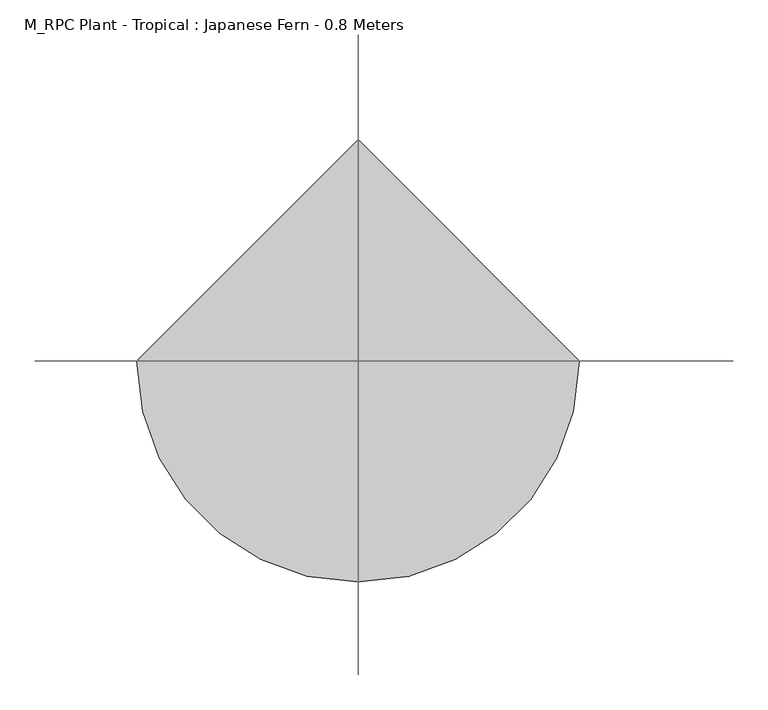
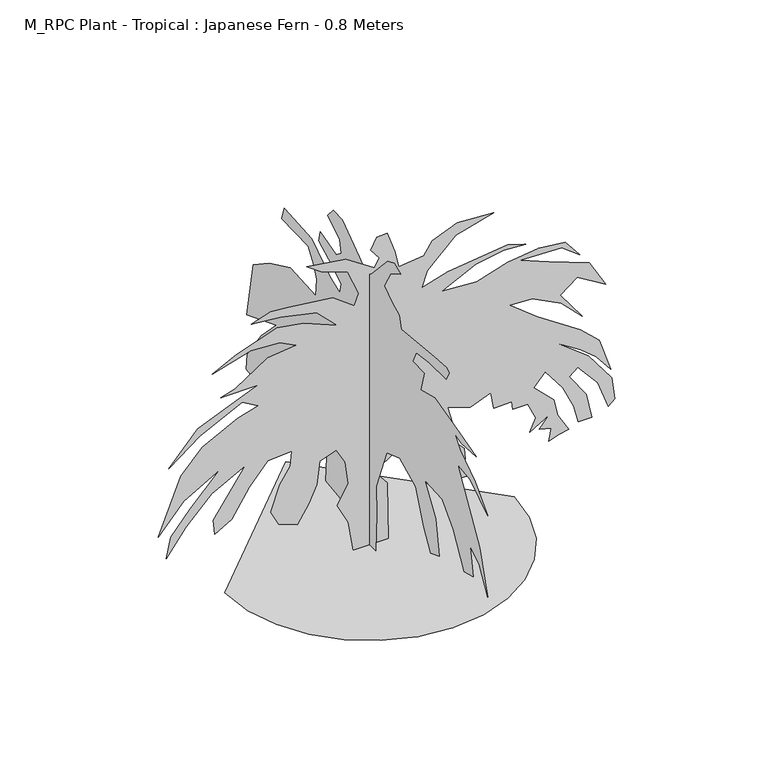
"""IFC4 building model written with IfcOpenShell, lengths in millimetres: geographic element geometry, M_RPC Plant - Tropical : Japanese Fern - 0.8 Meters."""

from ifc_helpers import new_model, si_unit, origin, place, context, project, spatial, triangles, source, transform, mapped, element, save


def m_rpc_plant_tropical_japanese_fern_0_8_meters_89f61e38(model_context):
    return source(origin(), model_context, "Body", "Tessellation", [
        triangles([(-356.9816259, 0.0, 2.46e-05), (-347.538961, -81.8417886, 2.46e-05), (-320.6483422, -157.0003733, 2.46e-05), (-278.4590569, -223.3224515, 2.46e-05), (-223.1257884, -278.6557201, 2.46e-05), (-156.8037101, -320.8450235, 2.46e-05), (-81.6451164, -347.7356423, 2.46e-05), (0.1966867, -357.1783072, 2.46e-05), (82.0384609, -347.7356423, 2.46e-05), (157.1970364, -320.8450235, 2.46e-05), (223.5191146, -278.6557201, 2.46e-05), (278.8523832, -223.3224515, 2.46e-05), (321.0417048, -157.0003733, 2.46e-05), (347.9323236, -81.8417886, 2.46e-05), (357.3749886, 3.12e-05, 2.46e-05), (0.1966242, 357.1783072, 2.46e-05), (-39.591288, 2.4e-05, 3.8e-06), (-52.3886082, 2.53e-05, 77.2092589), (-79.4701856, 2.33e-05, 129.9044073), (-51.8286088, 1.92e-05, 179.0246285), (-59.6237998, 1.61e-05, 237.2005651), (-81.0099172, 1.47e-05, 275.3224025), (-121.8640096, 1.74e-05, 260.7322683), (-129.4650627, 2.12e-05, 202.3781994), (-150.0026445, 2.47e-05, 159.3985009), (-177.3082362, 2.85e-05, 114.8257492), (-224.1652416, 2.95e-05, 132.5502668), (-243.9444304, 2.81e-05, 171.1790318), (-221.0799103, 2.33e-05, 234.4691003), (-195.0511394, 1.98e-05, 273.6130591), (-191.2119478, 1.74e-05, 311.3276902), (-250.2614867, 2.02e-05, 307.4210246), (-296.6350369, 2.54e-05, 254.2280142), (-339.5123071, 3.14e-05, 185.9592888), (-381.4722822, 3.47e-05, 161.1515734), (-385.2696158, 3.25e-05, 199.7619347), (-305.7070304, 2.23e-05, 313.25835), (-389.2322737, 2.86e-05, 269.5890678), (-451.6135314, 3.51e-05, 205.2877965), (-501.5068159, 4.12e-05, 139.8979924), (-490.5788492, 3.76e-05, 191.9816683), (-441.6242065, 3.21e-05, 249.0544201), (-368.8616057, 2.43e-05, 325.6103577), (-458.3148665, 3.13e-05, 274.3943886), (-521.6481374, 3.83e-05, 202.3696607), (-465.4295122, 2.75e-05, 342.7516442), (-412.306919, 2.18e-05, 399.0182679), (-325.1523188, 1.53e-05, 444.1942168), (-273.6057376, 1.22e-05, 459.1648873), (-314.0723265, 1.26e-05, 482.4155394), (-418.6162359, 2.03e-05, 430.012924), (-495.2054927, 2.71e-05, 372.3782879), (-423.1042251, 1.92e-05, 451.5675676), (-315.4003341, 1.18e-05, 496.7035117), (-275.4804052, 9.1e-06, 512.7808371), (-366.2136206, 1.31e-05, 512.5835017), (-331.2056557, 1.09e-05, 523.2341598), (-250.2614867, 4.2e-06, 575.8901027), (-180.8079499, 7e-07, 584.7194329), (-221.0799103, 1.2e-06, 605.0713883), (-292.4937199, 4.1e-06, 609.4207232), (-387.4135983, 9.9e-06, 581.7274281), (-328.4856545, 5.5e-06, 612.0154049), (-227.295374, -1e-06, 646.7967121), (-161.5869029, -3.2e-06, 635.7193359), (-78.621382, -4.8e-06, 600.674055), (-129.4533356, -5.6e-06, 651.5887161), (-219.3260566, -2.8e-06, 670.7326784), (-291.1150432, -1e-07, 678.0232944), (-243.6241556, -3.1e-06, 694.5326792), (-199.2876722, -4.8e-06, 690.5139565), (-89.7989701, -8.8e-06, 676.7513517), (-37.2379591, -8.7e-06, 637.1700468), (-25.5654385, -1.1e-05, 666.3513325), (-53.2067405, -1.36e-05, 730.9165775), (-118.8594782, -1.21e-05, 754.0578976), (-153.9631858, -1.22e-05, 780.1592113), (-58.1566019, -1.55e-05, 766.6525503), (12.3701786, -1.58e-05, 718.8793036), (24.5030987, -1.76e-05, 741.3032982), (3.6158409, -1.84e-05, 768.4872494), (18.7047597, -2.07e-05, 796.1618683), (43.7640938, -2.19e-05, 798.4898512), (62.816342, -1.95e-05, 744.3539114), (72.129132, -1.74e-05, 701.4126371), (134.0245409, -2.04e-05, 707.8552671), (155.3583768, -2.33e-05, 739.3059637), (216.6393747, -2.75e-05, 765.5672241), (307.1003683, -3.11e-05, 759.7325512), (213.1465828, -2.54e-05, 733.5272467), (143.1669335, -1.83e-05, 665.9780268), (130.1258781, -1.53e-05, 625.1620588), (193.29407, -1.93e-05, 645.9246723), (342.1190157, -2.69e-05, 663.433996), (386.0096143, -2.8e-05, 650.2686659), (331.6310294, -2.58e-05, 653.215361), (262.3572055, -2.2e-05, 640.2313425), (179.4618111, -1.6e-05, 599.1567421), (265.035058, -1.94e-05, 594.3860667), (342.0896934, -2.42e-05, 617.5967503), (417.9909471, -2.81e-05, 628.4153486), (483.3268573, -3.05e-05, 620.5620489), (520.1241752, -2.95e-05, 575.8901027), (475.7348788, -2.95e-05, 609.4687217), (372.9456588, -2.52e-05, 612.3860945), (441.3349073, -2.65e-05, 584.6447645), (542.8041498, -2.87e-05, 546.4048021), (584.2227699, -2.63e-05, 476.0742113), (513.9028253, -2.58e-05, 519.0714778), (472.0308898, -2.2e-05, 486.8048427), (525.9615005, -2e-05, 412.4742416), (473.4335295, -2.08e-05, 465.0022127), (402.3962957, -1.99e-05, 501.5674953), (346.6470097, -1.76e-05, 504.9195073), (415.0709218, -1.74e-05, 450.4102255), (520.5801793, -1.78e-05, 379.9196154), (568.2414416, -1.72e-05, 335.1356847), (596.0814211, -1.33e-05, 249.2213612), (560.7561427, -1.45e-05, 294.909034), (522.6121774, -1.47e-05, 326.2076686), (462.342891, -1.43e-05, 363.9543108), (540.550799, -1.42e-05, 304.5037063), (599.2467439, -1.21e-05, 226.7565805), (605.6067481, -9e-06, 169.6256927), (590.1587448, -7.5e-06, 155.6795782), (563.8974481, -1.05e-05, 225.714711), (514.2895022, -1.18e-05, 284.0770462), (493.1588516, -9.9e-06, 266.7677284), (536.2361641, -8.1e-06, 205.2771322), (549.3054608, -4.8e-06, 141.0889262), (516.425491, -3.3e-06, 140.2646579), (505.3241701, -5.5e-06, 185.108614), (477.6415575, -7.8e-06, 243.2032329), (434.3535748, -9.2e-06, 299.3437015), (405.9722766, -6.1e-06, 268.3197412), (455.9268946, -5.4e-06, 219.8784575), (465.4788915, -3.2e-06, 174.9152863), (492.2202098, -1.7e-06, 130.1460077), (468.8415496, -3e-07, 124.1884135), (442.7215596, 1.3e-06, 116.1070845), (449.5455617, -8e-07, 146.8782531), (419.662938, 0.0, 155.0435705), (444.2522438, -2.8e-06, 184.860882), (396.2229444, 1e-06, 156.0027779), (410.9322573, -1.6e-06, 188.0872839), (391.7616251, -3.2e-06, 229.804832), (353.6443296, -1.6e-06, 230.0109786), (351.7750033, -2.7e-06, 250.1848198), (307.1003683, -7e-07, 249.0597613), (300.2817075, -2.9e-06, 291.6023862), (248.7385418, 5e-07, 272.405066), (193.29407, 1.9e-06, 289.9143715), (210.8028487, 4.9e-06, 225.714711), (209.5596469, 6.7e-06, 196.5163297), (234.147899, 7.2e-06, 170.2702392), (237.0660348, 8.8e-06, 141.0889262), (219.1519212, 1.04e-05, 127.6382756), (249.9017521, 1.1e-05, 94.9585752), (191.3132679, 1.34e-05, 97.4711035), (201.263133, 1.05e-05, 139.9955973), (173.9058276, 1.05e-05, 159.8089046), (182.4415529, 8.6e-06, 185.1459482), (114.684288, 1.2e-05, 178.0643492), (99.9141775, 1.12e-05, 202.3696607), (152.4405135, 7.1e-06, 231.5509645), (87.6747175, 9.8e-06, 234.8944377), (12.4554318, 1.6e-05, 186.0566121), (44.4696966, 1.69e-05, 146.9251888), (47.3878233, 1.91e-05, 0.0), (0.1988968, 28.0250381, 3.7e-06), (0.1989024, 23.3153101, 131.4809371), (0.1989043, 63.1703357, 135.2526637), (0.1989031, 125.3580096, 45.104755), (0.1989061, 186.8720783, 53.6724779), (0.1989088, 182.1083611, 118.7774792), (0.1989112, 144.4259864, 212.5160617), (0.1989072, 143.3849253, 265.1541278), (0.1989091, 175.7563505, 275.9837175), (0.1989147, 237.6858916, 199.7619347), (0.198915, 302.7357001, 140.1214617), (0.1989165, 331.3730146, 147.3601187), (0.1989186, 325.3463476, 199.5424713), (0.1989213, 363.9222997, 223.1101825), (0.1989223, 429.8262348, 180.7067569), (0.1989222, 475.8741872, 131.4809371), (0.1989247, 526.6901261, 139.4206596), (0.1989263, 521.9248283, 180.7067569), (0.1989212, 463.1728912, 264.866936), (0.1989213, 397.7889462, 332.7090159), (0.1989246, 523.5141572, 283.9223863), (0.1989299, 495.7835097, 430.9862294), (0.1989289, 428.236906, 476.0608764), (0.1989268, 339.3143177, 517.3488358), (0.1989217, 228.4952462, 512.2821756), (0.1989235, 224.9824519, 557.0447777), (0.1989254, 238.2328241, 586.9834299), (0.198928, 261.7722666, 621.3780602), (0.198933, 375.8342906, 623.7380178), (0.198934, 364.7196347, 657.0846743), (0.1989285, 247.1213622, 649.612674), (0.1989229, 169.3534347, 598.4660866), (0.1989203, 125.6708085, 581.7007582), (0.1989213, 121.2033486, 608.4554114), (0.1989249, 174.1686204, 639.6180079), (0.1989278, 217.0427113, 661.8500084), (0.1989224, 209.1029888, 690.4313307), (0.1989186, 140.9505263, 671.9353666), (0.1989184, 120.1790834, 688.8446543), (0.1989201, 126.4332074, 719.3166315), (0.1989238, 178.9323558, 752.3619255), (0.1989239, 155.1134427, 779.3565714), (0.1989222, 117.0030872, 777.7672062), (0.1989167, 43.7690217, 725.5806387), (0.1989142, 11.282335, 699.1806513), (0.1989139, -10.6222293, 714.4366241), (0.1989141, -78.3121894, 787.2951857), (0.1989134, -106.8948288, 799.9992067), (0.1989117, -133.8897381, 787.2951857), (0.1989124, -91.4905729, 762.6498877), (0.1989115, -63.82447, 714.9192982), (0.198909, -97.1412363, 690.3886734), (0.1989071, -127.8788042, 676.3806622), (0.1989116, -136.2243976, 645.8900087), (0.1988998, -278.3917282, 660.2606432), (0.1988976, -330.7943436, 663.4366848), (0.1988968, -341.9089994, 655.4979979), (0.1989026, -329.2050147, 631.6793936), (0.1989057, -255.7989394, 630.9247158), (0.1989078, -201.4115251, 623.4394169), (0.1989071, -185.4035451, 591.3727332), (0.1989049, -234.4786928, 590.4820899), (0.1989033, -219.4389858, 537.8608106), (0.1989013, -279.9783864, 553.8714612), (0.1988956, -384.8262926, 526.9594774), (0.1988915, -456.2395572, 506.2314912), (0.1988942, -394.0155936, 503.9995053), (0.1988957, -365.7943148, 511.6901696), (0.1988935, -388.4636069, 482.6261733), (0.1988888, -452.284893, 439.6635704), (0.198884, -507.0528437, 383.9622828), (0.1988894, -430.8768974, 431.8128868), (0.198892, -378.3489627, 438.6928811), (0.1988872, -418.3222495, 368.7036212), (0.1988809, -472.1195472, 279.1570521), (0.1988809, -505.8634904, 170.2702392), (0.198879, -470.530182, 233.1083004), (0.1988817, -430.9435721, 256.6434736), (0.1988781, -444.5382365, 186.5443548), (0.1988855, -406.6475987, 176.1064927), (0.198885, -359.3756295, 258.5152162), (0.1988892, -311.2476806, 308.3676965), (0.1988927, -237.3971011, 313.25835), (0.1988874, -284.7437206, 241.0480229), (0.1988892, -298.5170441, 151.7734485), (0.1988901, -261.8053315, 136.5182659), (0.1988937, -232.8570984, 188.3064747), (0.1988926, -197.5672648, 272.0370652), (0.198897, -130.1718691, 304.5676922), (0.1988986, -73.5660583, 284.6663815), (0.1989018, -28.8695723, 170.457437), (0.1988986, -31.953834, 99.3204365), (0.1988944, -26.9829074, 2.55e-05)], [[15, 16, 1], [14, 15, 1], [14, 1, 2], [13, 14, 2], [13, 2, 3], [13, 3, 4], [12, 13, 4], [11, 12, 4], [11, 4, 5], [11, 5, 6], [11, 6, 7], [11, 7, 8], [11, 8, 9], [11, 9, 10], [110, 111, 112], [51, 52, 53], [61, 62, 63], [102, 103, 104], [94, 95, 96], [55, 56, 57], [88, 89, 90], [44, 45, 46], [117, 118, 119], [61, 63, 64], [68, 69, 70], [39, 40, 41], [107, 108, 109], [76, 77, 78], [39, 41, 42], [75, 76, 78], [38, 39, 42], [38, 42, 43], [60, 61, 64], [143, 144, 145], [93, 94, 96], [93, 96, 97], [93, 97, 98], [68, 70, 71], [37, 38, 43], [55, 57, 58], [157, 158, 159], [157, 159, 160], [75, 78, 79], [92, 93, 98], [74, 75, 79], [67, 68, 71], [67, 71, 72], [110, 112, 113], [139, 140, 141], [87, 88, 90], [87, 90, 91], [86, 87, 91], [117, 119, 120], [116, 117, 120], [116, 120, 121], [115, 116, 121], [101, 102, 104], [101, 104, 105], [100, 101, 105], [106, 107, 109], [34, 35, 36], [141, 142, 143], [43, 44, 46], [43, 46, 47], [124, 125, 126], [123, 124, 126], [122, 123, 126], [122, 126, 127], [34, 36, 37], [33, 34, 37], [32, 33, 37], [60, 64, 65], [59, 60, 65], [137, 138, 139], [137, 139, 141], [137, 141, 143], [136, 137, 143], [121, 122, 127], [50, 51, 53], [50, 53, 54], [66, 67, 72], [66, 72, 73], [106, 109, 110], [106, 110, 113], [129, 130, 131], [129, 131, 132], [129, 132, 133], [128, 129, 133], [128, 133, 134], [43, 47, 48], [37, 43, 48], [105, 106, 113], [105, 113, 114], [100, 105, 114], [99, 100, 114], [59, 65, 66], [163, 164, 165], [162, 163, 165], [168, 169, 17], [168, 17, 18], [168, 18, 19], [168, 19, 20], [167, 168, 20], [167, 20, 21], [146, 147, 148], [121, 127, 128], [121, 128, 134], [85, 86, 91], [148, 149, 150], [37, 48, 49], [32, 37, 49], [31, 32, 49], [85, 91, 92], [25, 26, 27], [25, 27, 28], [25, 28, 29], [24, 25, 29], [24, 29, 30], [23, 24, 30], [23, 30, 31], [136, 143, 145], [135, 136, 145], [135, 145, 146], [135, 146, 148], [82, 83, 84], [81, 82, 84], [80, 81, 84], [80, 84, 85], [79, 80, 85], [50, 54, 55], [49, 50, 55], [160, 161, 162], [156, 157, 160], [155, 156, 160], [155, 160, 162], [154, 155, 162], [154, 162, 165], [153, 154, 165], [152, 153, 165], [74, 79, 85], [74, 85, 92], [73, 74, 92], [166, 167, 21], [55, 58, 59], [166, 21, 22], [152, 165, 166], [135, 148, 150], [134, 135, 150], [121, 134, 150], [115, 121, 150], [114, 115, 150], [114, 150, 151], [114, 151, 152], [99, 114, 152], [98, 99, 152], [98, 152, 166], [98, 166, 22], [92, 98, 22], [73, 92, 22], [66, 73, 22], [59, 66, 22], [55, 59, 22], [49, 55, 22], [31, 49, 22], [23, 31, 22], [244, 245, 246], [239, 240, 241], [234, 235, 236], [234, 236, 237], [233, 234, 237], [238, 239, 241], [238, 241, 242], [217, 218, 219], [216, 217, 219], [189, 190, 191], [244, 246, 247], [215, 216, 219], [215, 219, 220], [197, 198, 199], [197, 199, 200], [230, 231, 232], [189, 191, 192], [209, 210, 211], [209, 211, 212], [209, 212, 213], [208, 209, 213], [197, 200, 201], [196, 197, 201], [195, 196, 201], [243, 244, 247], [262, 170, 171], [261, 262, 171], [260, 261, 171], [205, 206, 207], [204, 205, 207], [203, 204, 207], [185, 186, 187], [184, 185, 187], [184, 187, 188], [183, 184, 188], [183, 188, 189], [173, 174, 175], [172, 173, 175], [172, 175, 176], [247, 248, 249], [247, 249, 250], [243, 247, 250], [243, 250, 251], [242, 243, 251], [254, 255, 256], [253, 254, 256], [253, 256, 257], [252, 253, 257], [225, 226, 227], [224, 225, 227], [224, 227, 228], [223, 224, 228], [223, 228, 229], [223, 229, 230], [180, 181, 182], [179, 180, 182], [189, 192, 193], [189, 193, 194], [252, 257, 258], [203, 207, 208], [242, 251, 252], [208, 213, 214], [203, 208, 214], [183, 189, 194], [182, 183, 194], [179, 182, 194], [178, 179, 194], [177, 178, 194], [195, 201, 202], [194, 195, 202], [177, 194, 202], [237, 238, 242], [237, 242, 252], [233, 237, 252], [232, 233, 252], [232, 252, 258], [230, 232, 258], [230, 258, 259], [223, 230, 259], [221, 222, 223], [221, 223, 259], [220, 221, 259], [215, 220, 259], [214, 215, 259], [203, 214, 259], [202, 203, 259], [177, 202, 259], [177, 259, 260], [176, 177, 260], [172, 176, 260], [172, 260, 171]], closed=False),
    ])


if __name__ == "__main__":
    model = new_model("IFC4")
    model_context = context("Model", 3, world=origin())
    ifc_project = project(units=[si_unit("LENGTHUNIT", "METRE", prefix="MILLI")], contexts=[model_context])
    site = spatial("IfcSite", under=ifc_project)
    building = spatial("IfcBuilding", under=site)
    placement = place(None, origin())
    m_rpc_plant_tropical_japanese_fern_0_8_meters_shape = m_rpc_plant_tropical_japanese_fern_0_8_meters_89f61e38(model_context)
    element("IfcGeographicElement", 1, ObjectType="M_RPC Plant - Tropical : Japanese Fern - 0.8 Meters", at=placement, inside=building, context=model_context, shape_type="MappedRepresentation", body=[
        mapped(m_rpc_plant_tropical_japanese_fern_0_8_meters_shape, transform((0.0, 0.0, 0.0), x_axis=(1.0, 0.0, 0.0), y_axis=(0.0, 1.0, 0.0), z_axis=(0.0, 0.0, 1.0))),
    ])
    save(model, "model.ifc")

# Revit data of these elements
# Type "M_RPC Plant - Tropical : Japanese Fern - 0.8 Meters"
#   built-in parameter 1005198 = "{2, 15},{39, RPC-16-G1GK-JAPX-7J4P-Q000-ST1L-LVER-AU},{1, 0},{1, 0},{2, 35},{1, 8},{5, Color},{1, 0},{1, 0},{3, 0.8},{3, 0.8},{3, 0.8},{1, 8},{7, BBoxMin},{1, 0},{1, 0},{1, 0},{1, 0},{1, 0},{1, 8},{7, BBoxMax},{1, 0},{1, 0},{1, 0},{1, 0},{1, 0},{2, 11},{9, RPCTypeId},{1, 0},{1, 0},{39, RPC-16-G1GK-JAPX-7J4P-Q000-ST1L-LVER-AU},{1, 6},{14, RPCPlantHeight},{1, 0},{1, 0},{7, 2.62467},{2, 11},{7, keyword},{1, 0},{1, 0},{53, :Geometry:RPC:Japanese Fern:plant:small:japanese fern},{2, 11},{8, category},{1, 0},{1, 0},{17, :Shrubs [General]},{2, 11},{12, LocalizedUID},{1, 0},{1, 0},{13, Japanese Fern},{2, 14},{6, Height},{1, 0},{1, 0},{7, 2.62467},{1, 2},{16, Cast Reflections},{1, 0},{1, 0},{1, 0},{1, 2},{12, Cast Shadows},{1, 0},{1, 0},{1, 1},{1, 2},{9, Lock View},{1, 0},{1, 0},{1, 0},{1, 4},{5, ViewC},{1, 0},{1, 0},{1, 0},{2, 11},{20, AdvancedUIDefinition},{1, 0},{1, 0},{0, },{2, 11},{10, AssetLibID},{1, 0},{1, 0},{36, 4D3F6E72-3F99-4203-98E9-AF80B3C7A7A4},{2, 11},{10, BaseSchema},{1, 0},{1, 0},{9, RPCSchema},{2, 11},{12, ExchangeGUID},{1, 0},{1, 0},{0, },{1, 2},{6, Hidden},{1, 0},{1, 0},{1, 0},{1, 4},{11, RPCCategory},{1, 0},{1, 0},{1, 0},{2, 11},{8, RPCImage},{1, 0},{1, 0},{0, },{1, 4},{13, SchemaVersion},{1, 0},{1, 0},{1, 4},{2, 11},{12, UIDefinition},{1, 0},{1, 0},{0, },{2, 11},{6, UIName},{1, 0},{1, 0},{39, RPC-16-G1GK-JAPX-7J4P-Q000-ST1L-LVER-AU},{2, 11},{11, VersionGUID},{1, 0},{1, 0},{9, RPCSchema},{2, 11},{9, assettype},{1, 0},{1, 0},{11, RPCGeometry},{2, 11},{11, description},{1, 0},{1, 0},{0, },{2, 11},{9, localname},{1, 0},{1, 0},{3, RPC},{2, 11},{9, localtype},{1, 0},{1, 0},{3, RPC},{1, 4},{8, revision},{1, 0},{1, 0},{1, 1},{2, 11},{9, thumbnail},{1, 0},{1, 0},{0, },{1, 4},{7, version},{1, 0},{1, 0},{1, 1},{1, 2},{20, RPC_Cast Reflections},{1, 0},{1, 0},{1, 1},{1, 2},{16, RPC_Cast Shadows},{1, 0},{1, 0},{1, 1},{1, 2},{13, RPC_Lock View},{1, 0},{1, 0},{1, 0},{1, 4},{9, RPC_ViewC},{1, 0},{1, 0},{1, 0},{21, assetlibrary_base.fbx},{1, 5},"
#   built-in parameter 1005195 = "RPC-16-G1GK-JAPX-7J4P-Q000-ST1L-LVER-AU"
#   Type Comments = "Japanese Fern"
#   Height = 0.8 m
#   Description = (empty or 0)
#   Default Elevation = 0
